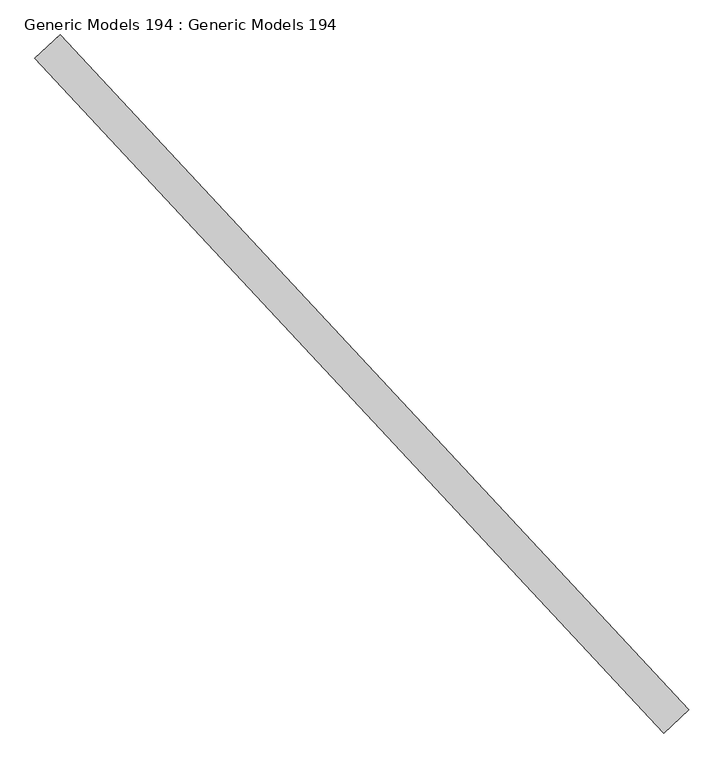
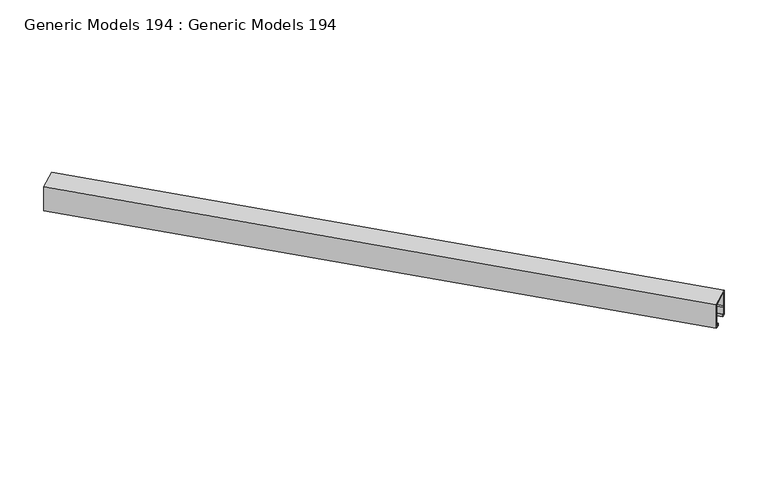
"""IFC4 building model written with IfcOpenShell, lengths in millimetres: proxy geometry, Generic Models 194 : Generic Models 194."""

from ifc_helpers import new_model, si_unit, frame, origin, place, context, project, spatial, polyline, outline, extrude, source, transform, mapped, element, save


def generic_models_194_generic_models_194_ab40d47e(model_context):
    return source(origin(), model_context, "Body", "SweptSolid", [
        extrude(outline(polyline([(0.0, 0.0), (6.35, 0.0), (6.35, -10.8), (-63.5, -10.8), (-63.5, 52.7), (6.35, 52.7), (6.35, 40.0), (0.0, 40.0), (0.0, 41.5875), (4.7625, 41.5875), (4.7625, 51.1125), (-61.9125, 51.1125), (-61.9125, -9.2125), (-19.9283243, -9.2125), (-19.9283243, -1.5875), (0.0, -1.5875), (0.0, 0.0)])), frame((-409.2964332, -19867.6933881, 2590.8), z_axis=(-0.681998360062497, 0.7313537016191719, 0.0), x_axis=(0.0, 0.0, -1.0)), (0.0, 0.0, 1.0), 1701.8),
    ])


if __name__ == "__main__":
    model = new_model("IFC4")
    model_context = context("Model", 3, world=origin())
    ifc_project = project(units=[si_unit("LENGTHUNIT", "METRE", prefix="MILLI")], contexts=[model_context])
    site = spatial("IfcSite", under=ifc_project)
    building = spatial("IfcBuilding", under=site)
    placement = place(None, origin())
    generic_models_194_generic_models_194_shape = generic_models_194_generic_models_194_ab40d47e(model_context)
    element("IfcBuildingElementProxy", 1, Name="Generic Models 194 : Generic Models 194", ObjectType="Generic Models 194 : Generic Models 194", at=placement, inside=building, context=model_context, shape_type="MappedRepresentation", body=[
        mapped(generic_models_194_generic_models_194_shape, transform((0.0, 0.0, 0.0), x_axis=(1.0, 0.0, 0.0), y_axis=(0.0, 1.0, 0.0), z_axis=(0.0, 0.0, 1.0))),
    ])
    save(model, "model.ifc")

# Revit data of these elements
# Element 1 (IfcBuildingElementProxy, "Generic Models 194 : Generic Models 194")
#   Materials on its faces: "EXISTING STOREFRONT"
# Materials
#   "EXISTING STOREFRONT": class "Metal", colour RGB 244 244 244, transparency 0, Description = "Aluminum 6061", Cost = 0
